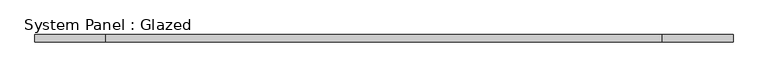
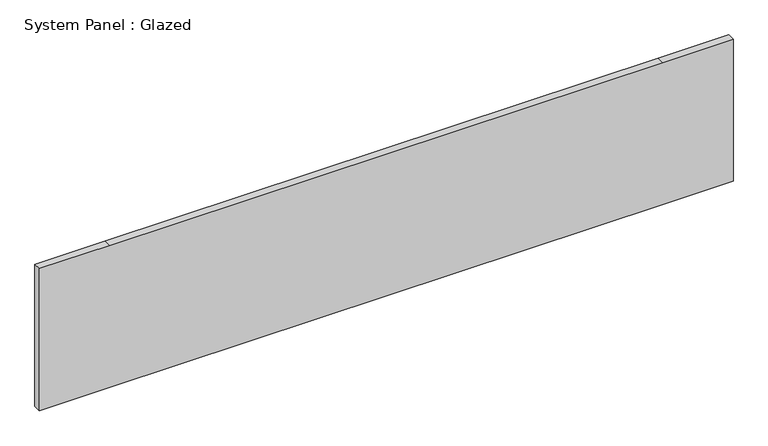
"""IFC4 building model written with IfcOpenShell, lengths in millimetres: plate geometry, System Panel : Glazed."""

from ifc_helpers import new_model, si_unit, frame, origin, place, context, project, spatial, polyline, outline, extrude, source, transform, mapped, element, save


def system_panel_glazed_5ffb59d1(model_context):
    return source(origin(), model_context, "Body", "SweptSolid", [
        extrude(outline(polyline([(0.0, -1187.45), (0.0, -946.15), (0.0, 946.15), (0.0, 1187.45), (514.35, 1187.45), (514.35, 946.15), (514.35, -946.15), (514.35, -1187.45), (0.0, -1187.45)])), frame((0.0, -44.45, 0.0), z_axis=(0.0, 1.0, 0.0), x_axis=(0.0, 0.0, 1.0)), (0.0, 0.0, 1.0), 25.4),
    ])


if __name__ == "__main__":
    model = new_model("IFC4")
    model_context = context("Model", 3, world=origin())
    ifc_project = project(units=[si_unit("LENGTHUNIT", "METRE", prefix="MILLI")], contexts=[model_context])
    site = spatial("IfcSite", under=ifc_project)
    building = spatial("IfcBuilding", under=site)
    placement = place(None, origin())
    system_panel_glazed_shape = system_panel_glazed_5ffb59d1(model_context)
    element("IfcPlate", 1, ObjectType="System Panel : Glazed", at=placement, inside=building, context=model_context, shape_type="MappedRepresentation", body=[
        mapped(system_panel_glazed_shape, transform((0.0, 0.0, 0.0), x_axis=(1.0, 0.0, 0.0), y_axis=(0.0, 1.0, 0.0), z_axis=(0.0, 0.0, 1.0))),
    ])
    save(model, "model.ifc")

# Revit data of these elements
# Element 1 (IfcPlate, "System Panel : Glazed")
#   Materials on its faces: "Glass"
# Materials
#   "Glass": class "Glass", colour RGB 0 128 192, transparency 0.75
